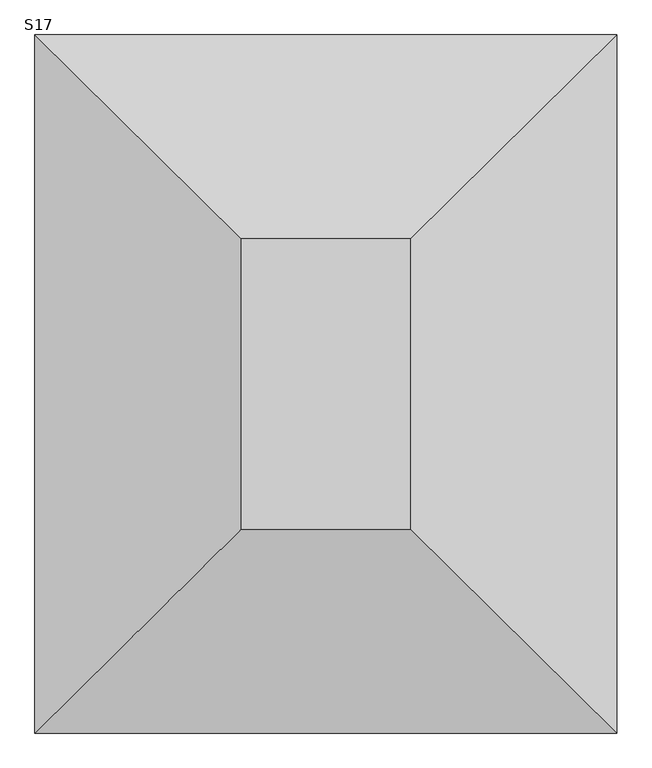
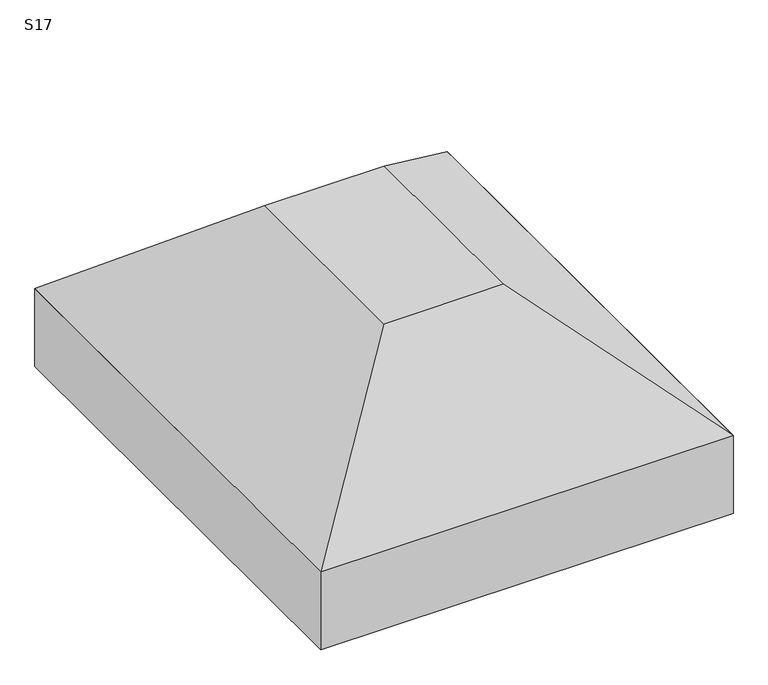
"""IFC4 building model written with IfcOpenShell, lengths in millimetres: fastener geometry, TQS - Sapata : S17."""

import ifcopenshell
import ifcopenshell.guid

model = None  # the IFC model being written
_history = None  # IfcOwnerHistory: only IFC2X3 demands one
_inside = {}  # id of a spatial element -> (the spatial element, [elements in it])
_under = {}  # id of a project, library or spatial element -> (it, [spatial elements below it])
_declared = {}  # id of a project -> (the project, [libraries it declares])
_typed = {}  # id of a type object -> (the type object, [elements of that type])
_made_of = {}  # id of a material, layer set ... -> (it, [elements and type objects made of it])


def new_model(schema):
    """Start an empty IFC model of exactly this schema.

    Asked for "IFC4X3", IfcOpenShell would pick the latest addendum, in which some entities
    have other attributes; the version numbers below select the first issue.
    IFC2X3 requires an IfcOwnerHistory on every rooted entity: one is made here for all.
    """
    global model, _history
    if schema == "IFC4X3":
        model = ifcopenshell.file(schema_version=(4, 3, 0, 0))
    else:
        model = ifcopenshell.file(schema=schema)
    _inside.clear()
    _under.clear()
    _declared.clear()
    _typed.clear()
    _made_of.clear()
    _history = None
    if model.schema == "IFC2X3":
        org = make("IfcOrganization", Name="unknown")
        user = make(
            "IfcPersonAndOrganization",
            ThePerson=make("IfcPerson", FamilyName="unknown"),
            TheOrganization=org,
        )
        app = make(
            "IfcApplication",
            ApplicationDeveloper=org,
            Version="unknown",
            ApplicationFullName="unknown",
            ApplicationIdentifier="unknown",
        )
        _history = make(
            "IfcOwnerHistory",
            OwningUser=user,
            OwningApplication=app,
            ChangeAction="ADDED",
            CreationDate=0,
        )
    return model


def make(cls, **values):
    """One entity of the class cls with the attributes given. An attribute that is None is left unset."""
    return model.create_entity(
        cls, **{name: value for name, value in values.items() if value is not None}
    )


def rooted(cls, **values):
    """An entity with a GlobalId (a new one), such as an element, a storey or a relation."""
    return make(cls, GlobalId=ifcopenshell.guid.new(), OwnerHistory=_history, **values)


def si_unit(unit_type, name, prefix=None):
    """IfcSIUnit, for example si_unit("LENGTHUNIT", "METRE", prefix="MILLI")."""
    return make("IfcSIUnit", UnitType=unit_type, Prefix=prefix, Name=name)


def assignment(units):
    """IfcUnitAssignment: the units of a project."""
    return None if units is None else make("IfcUnitAssignment", Units=units)


def point(xyz):
    """IfcCartesianPoint."""
    return None if xyz is None else make("IfcCartesianPoint", Coordinates=xyz)


def direction(xyz):
    """IfcDirection."""
    return None if xyz is None else make("IfcDirection", DirectionRatios=xyz)


def frame(location, z_axis=None, x_axis=None):
    """IfcAxis2Placement3D, a coordinate frame: its origin and axes. An axis left out is left unset."""
    return make(
        "IfcAxis2Placement3D",
        Location=point(location),
        Axis=direction(z_axis),
        RefDirection=direction(x_axis),
    )


def origin():
    """The frame at (0, 0, 0) with its axes left unset."""
    return frame((0.0, 0.0, 0.0))


def place(relative_to, where):
    """IfcLocalPlacement: puts the frame where relative to a parent placement (None: the world)."""
    return make(
        "IfcLocalPlacement", PlacementRelTo=relative_to, RelativePlacement=where
    )


def context(
    kind, dimensions, precision=None, world=None, true_north=None, identifier=None
):
    """IfcGeometricRepresentationContext, for example the 3D "Model" context."""
    return make(
        "IfcGeometricRepresentationContext",
        ContextIdentifier=identifier,
        ContextType=kind,
        CoordinateSpaceDimension=dimensions,
        Precision=precision,
        WorldCoordinateSystem=world,
        TrueNorth=true_north,
    )


def project(units=None, contexts=None):
    """IfcProject with its units and contexts."""
    return rooted(
        "IfcProject",
        Name="project",
        RepresentationContexts=contexts,
        UnitsInContext=assignment(units),
    )


def spatial(cls, under=None, at=None, **own):
    """A site, building, storey or space (cls), placed at a placement, below another one or the project."""
    s = rooted(cls, ObjectPlacement=at, **own)
    if under is not None:
        _under.setdefault(under.id(), (under, []))[1].append(s)
    return s


def polyline(points):
    """IfcPolyline through the points."""
    return make("IfcPolyline", Points=[point(p) for p in points])


def outline(outer, holes=None, kind="AREA"):
    """IfcArbitraryClosedProfileDef: a profile drawn as a closed curve; with holes, ...WithVoids."""
    if holes is None:
        return make("IfcArbitraryClosedProfileDef", ProfileType=kind, OuterCurve=outer)
    return make(
        "IfcArbitraryProfileDefWithVoids",
        ProfileType=kind,
        OuterCurve=outer,
        InnerCurves=holes,
    )


def extrude(swept, where, along, depth):
    """IfcExtrudedAreaSolid: the profile swept, set in the frame where, extruded along a direction by depth."""
    return make(
        "IfcExtrudedAreaSolid",
        SweptArea=swept,
        Position=where,
        ExtrudedDirection=direction(along),
        Depth=depth,
    )


def faces_of(points, faces, orient=None, outer=None):
    """IfcFace entities. A face is a list of loops; a loop is a list of indices into points, from 0.

    orient and outer hold one flag for each loop. By default every Orientation is true, the
    first loop of a face is its IfcFaceOuterBound and the others are IfcFaceBound.
    """
    made = []
    for i, loops in enumerate(faces):
        bounds = []
        for j, loop in enumerate(loops):
            is_outer = j == 0 if outer is None else outer[i][j]
            bounds.append(
                make(
                    "IfcFaceOuterBound" if is_outer else "IfcFaceBound",
                    Bound=make("IfcPolyLoop", Polygon=[points[k] for k in loop]),
                    Orientation=True if orient is None else orient[i][j],
                )
            )
        made.append(make("IfcFace", Bounds=bounds))
    return made


def faceted_brep(points, faces, orient=None, outer=None, voids=None):
    """IfcFacetedBrep: a solid bounded by flat faces; with voids (closed shells), ...WithVoids."""
    shared = [point(p) for p in points]
    hull = make("IfcClosedShell", CfsFaces=faces_of(shared, faces, orient, outer))
    if voids is None:
        return make("IfcFacetedBrep", Outer=hull)
    return make(
        "IfcFacetedBrepWithVoids",
        Outer=hull,
        Voids=[
            make(cls, CfsFaces=faces_of(shared, fs, o, b)) for cls, fs, o, b in voids
        ],
    )


def shape(context_of_items, identifier, shape_type, items):
    """IfcShapeRepresentation: the items that make up one representation, for example the "Body"."""
    return make(
        "IfcShapeRepresentation",
        ContextOfItems=context_of_items,
        RepresentationIdentifier=identifier,
        RepresentationType=shape_type,
        Items=items,
    )


def source(mapping_origin, context_of_items, identifier, shape_type, items):
    """IfcRepresentationMap: a shape defined once, which mapped items show again and again."""
    return make(
        "IfcRepresentationMap",
        MappingOrigin=mapping_origin,
        MappedRepresentation=shape(context_of_items, identifier, shape_type, items),
    )


def transform(
    local_origin,
    x_axis=None,
    y_axis=None,
    z_axis=None,
    scale=None,
    scale2=None,
    scale3=None,
    uniform=True,
):
    """IfcCartesianTransformationOperator3D, or its non-uniform kind. x_axis, y_axis, z_axis: its Axis1, 2, 3."""
    if uniform:
        return make(
            "IfcCartesianTransformationOperator3D",
            Axis1=direction(x_axis),
            Axis2=direction(y_axis),
            LocalOrigin=point(local_origin),
            Scale=scale,
            Axis3=direction(z_axis),
        )
    return make(
        "IfcCartesianTransformationOperator3DnonUniform",
        Axis1=direction(x_axis),
        Axis2=direction(y_axis),
        LocalOrigin=point(local_origin),
        Scale=scale,
        Axis3=direction(z_axis),
        Scale2=scale2,
        Scale3=scale3,
    )


def mapped(mapping_source, mapping_target):
    """IfcMappedItem: shows the shape of a source again, moved by a transform."""
    return make(
        "IfcMappedItem", MappingSource=mapping_source, MappingTarget=mapping_target
    )


def made_of(thing, what):
    """Note that an element or type object is made of a material, layer set ...; save() writes the relation."""
    if what is not None:
        _made_of.setdefault(what.id(), (what, []))[1].append(thing)
    return thing


def element(
    cls,
    number,
    at=None,
    inside=None,
    cuts=None,
    type_object=None,
    material=None,
    context=None,
    identifier="Body",
    shape_type=None,
    held_by="IfcProductDefinitionShape",
    body=None,
    shapes=None,
    **own,
):
    """One element of the class cls, such as IfcWall. Its Tag is "e" and its number.

    at: its placement. inside: the storey or other place that contains it. cuts: it is an
    opening in that element (IfcRelVoidsElement). A single representation is given by context,
    identifier, shape_type and body (its items); several are given by shapes. held_by: the class
    of the entity that holds the representations. save() writes the other relations.
    """
    e = rooted(cls, Tag="e%d" % number, ObjectPlacement=at, **own)
    if body is not None:
        shapes = [shape(context, identifier, shape_type, body)]
    if shapes is not None:
        e.Representation = make(held_by, Representations=shapes)
    if inside is not None:
        _inside.setdefault(inside.id(), (inside, []))[1].append(e)
    if cuts is not None:
        rooted(
            "IfcRelVoidsElement", RelatingBuildingElement=cuts, RelatedOpeningElement=e
        )
    if type_object is not None:
        _typed.setdefault(type_object.id(), (type_object, []))[1].append(e)
    return made_of(e, material)


def aggregate(whole, parts):
    """IfcRelAggregates: a whole, such as a stair, and the parts it consists of."""
    return rooted("IfcRelAggregates", RelatingObject=whole, RelatedObjects=parts)


def save(model, path):
    """Write the relations noted so far, then the file.

    IfcRelAggregates (storeys below a building ...), IfcRelContainedInSpatialStructure (elements
    in a storey), IfcRelDefinesByType, IfcRelAssociatesMaterial and IfcRelDeclares: one each for
    every whole, place, type object, material and project.
    """
    for whole, parts in _under.values():
        aggregate(whole, parts)
    for where, things in _inside.values():
        rooted(
            "IfcRelContainedInSpatialStructure",
            RelatedElements=things,
            RelatingStructure=where,
        )
    for kind, things in _typed.values():
        rooted("IfcRelDefinesByType", RelatedObjects=things, RelatingType=kind)
    for what, things in _made_of.values():
        rooted("IfcRelAssociatesMaterial", RelatedObjects=things, RelatingMaterial=what)
    for by, libraries in _declared.values():
        rooted("IfcRelDeclares", RelatingContext=by, RelatedDefinitions=libraries)
    model.write(path)


def s17_fc997501(model_context):
    return source(origin(), model_context, "Body", "SolidModel", [
        faceted_brep([(-55.0, 50.0, 0.0), (-345.0, 50.0, 0.0), (-345.0, -450.0, 0.0), (-55.0, -450.0, 0.0), (300.0, 400.0, -300.0), (300.0, -800.0, -300.0), (-700.0, -800.0, -300.0), (-700.0, 400.0, -300.0)], [[[0, 1, 2, 3]], [[4, 5, 6, 7]], [[4, 7, 1, 0]], [[7, 6, 2, 1]], [[6, 5, 3, 2]], [[5, 4, 0, 3]]]),
        extrude(outline(polyline([(300.0, 400.0), (300.0, -800.0), (-700.0, -800.0), (-700.0, 400.0), (300.0, 400.0)])), frame((0.0, 0.0, -500.0), z_axis=(0.0, 0.0, 1.0), x_axis=(1.0, 0.0, 0.0)), (0.0, 0.0, 1.0), 200.0),
    ])


if __name__ == "__main__":
    model = new_model("IFC4")
    model_context = context("Model", 3, world=origin())
    ifc_project = project(units=[si_unit("LENGTHUNIT", "METRE", prefix="MILLI")], contexts=[model_context])
    site = spatial("IfcSite", under=ifc_project)
    building = spatial("IfcBuilding", under=site)
    placement = place(None, origin())
    s17_shape = s17_fc997501(model_context)
    element("IfcFastener", 1, ObjectType="TQS - Sapata : S17", at=placement, inside=building, context=model_context, shape_type="MappedRepresentation", body=[
        mapped(s17_shape, transform((0.0, 0.0, 0.0), x_axis=(1.0, 0.0, 0.0), y_axis=(0.0, 1.0, 0.0), z_axis=(0.0, 0.0, 1.0))),
    ])
    save(model, "model.ifc")

# Revit data of these elements
# Type "TQS - Sapata : S17"
#   TY = 0.50 m
#   TX = 0.29 m
#   HS = 0.50 m
#   H0 = 0.20 m
#   EXCYABS = 0.60 m
#   EXCY = 0.00 m
#   EXCXABS = 0.50 m
#   EXCX = 0.00 m
#   DIMY = 1.20 m
#   DIMX = 1.00 m
#   Material estrutural = Concreto - Concreto concretado no local
#   Width = 0
#   Length = 0
# Element 1 (IfcFastener, "TQS - Sapata : S17")
#   Materials on its faces: "Concreto - Concreto concretado no local"
# Materials
#   "Concreto - Concreto concretado no local": class "Concreto", colour RGB 192 192 192, transparency 0
